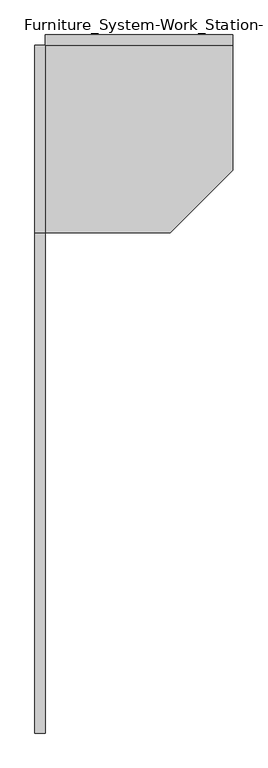
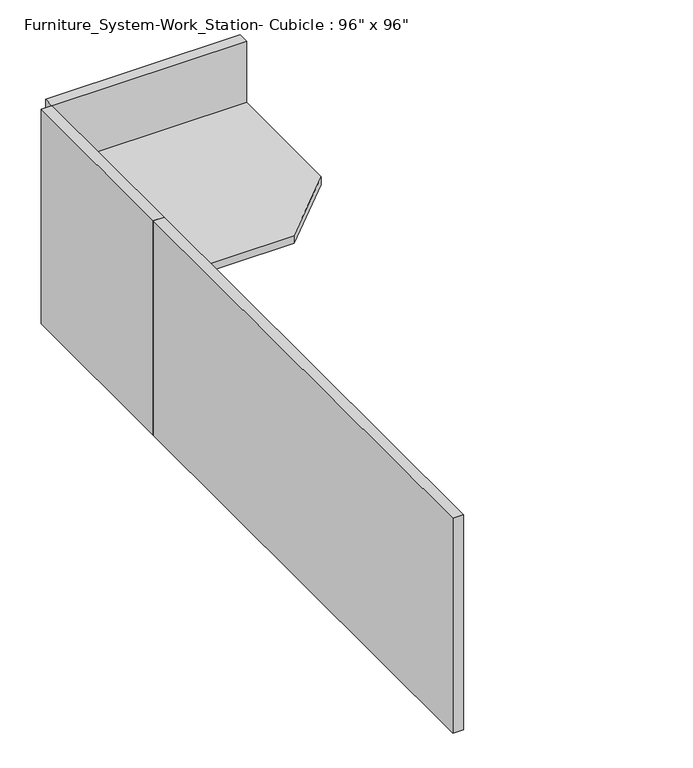
"""IFC4 building model written with IfcOpenShell, lengths in millimetres: furniture geometry."""

from ifc_helpers import new_model, si_unit, frame, origin, origin_with_axes, place, context, project, spatial, polyline, outline, extrude, source, transform, mapped, element, save


def furniture_2ff4602c(model_context):
    return source(origin(), model_context, "Body", "SweptSolid", [
        extrude(outline(polyline([(-80.9317522, -545.8230076), (833.4682478, -545.8230076), (833.4682478, -1155.4230076), (528.6682478, -1460.2230076), (-80.9317522, -1460.2230076), (-80.9317522, -545.8230076)])), frame((0.0, 0.0, 723.9), z_axis=(0.0, 0.0, 1.0), x_axis=(1.0, 0.0, 0.0)), (0.0, 0.0, 1.0), 38.1),
        extrude(outline(polyline([(833.4682478, -545.8230076), (-80.9317522, -545.8230076), (-80.9317522, -495.0230076), (833.4682478, -495.0230076), (833.4682478, -545.8230076)])), origin_with_axes(), (0.0, 0.0, 1.0), 1066.8),
        extrude(outline(polyline([(-80.9317522, -1460.2230076), (-131.7317522, -1460.2230076), (-131.7317522, -545.8230076), (-80.9317522, -545.8230076), (-80.9317522, -1460.2230076)])), origin_with_axes(), (0.0, 0.0, 1.0), 1066.8),
        extrude(outline(polyline([(-80.9317522, -3898.6230076), (-131.7317522, -3898.6230076), (-131.7317522, -1460.2230076), (-80.9317522, -1460.2230076), (-80.9317522, -3898.6230076)])), origin_with_axes(), (0.0, 0.0, 1.0), 1066.8),
    ])


if __name__ == "__main__":
    model = new_model("IFC4")
    model_context = context("Model", 3, world=origin())
    ifc_project = project(units=[si_unit("LENGTHUNIT", "METRE", prefix="MILLI")], contexts=[model_context])
    site = spatial("IfcSite", under=ifc_project)
    building = spatial("IfcBuilding", under=site)
    placement = place(None, origin())
    furniture_shape = furniture_2ff4602c(model_context)
    element("IfcFurniture", 1, ObjectType="Furniture_System-Work_Station- Cubicle : 96\" x 96\"", at=placement, inside=building, context=model_context, shape_type="MappedRepresentation", body=[
        mapped(furniture_shape, transform((0.0, 0.0, 0.0), x_axis=(1.0, 0.0, 0.0), y_axis=(0.0, 1.0, 0.0), z_axis=(0.0, 0.0, 1.0))),
    ])
    save(model, "model.ifc")

# Revit data of these elements
# Project information
#   Project Issue Date = "Issue Date"
#   Project Status = "Project Status"
#   Client Name = "Owner"
#   Project Address = "Enter address here"
#   Project Name = "Project Name"
#   Project Number = "Project Number"
# Type "Furniture_System-Work_Station- Cubicle : 96\" x 96\""
#   Assembly Code = "E2020"
#   Desktop Height = 2' - 6"
#   Desktop1 Width = 2' - 0"
#   Desktop2 Width = 2' - 0"
#   Panel Height = 3' - 6"
#   Panel1 Length = 8' - 0"
#   Panel2 Length = 0' - 0"
#   Cube Panel Material = Textile - Light Gray
#   Work Top Material = Laminate - Ivory,Matte
#   Default Elevation = 0
# Element 1 (IfcFurniture, "Furniture_System-Work_Station- Cubicle : 96\" x 96\"")
#   Materials on its faces: "Textile - Light Gray", "Laminate - Ivory,Matte"
# Materials
#   "Textile - Light Gray": class "Unassigned", colour RGB 204 204 204, transparency 0
#   "Laminate - Ivory,Matte": class "Unassigned", colour RGB 127 127 127, transparency 0, Comments = "Rendering appearance not upgraded "
